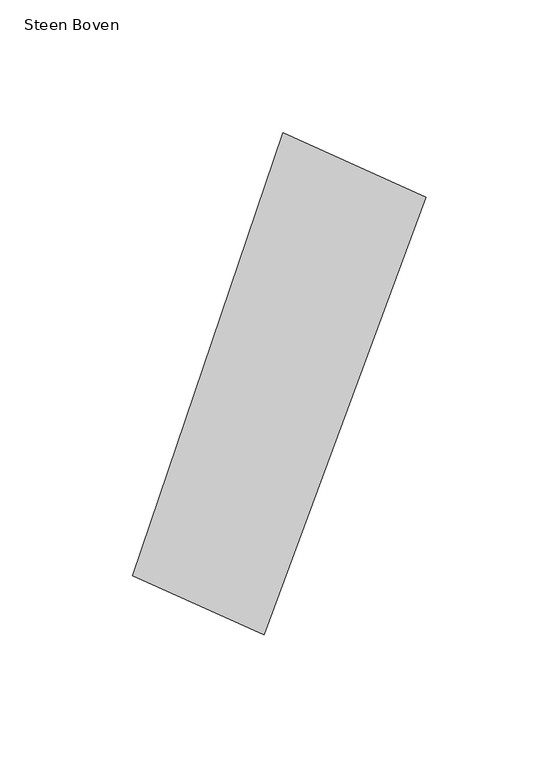
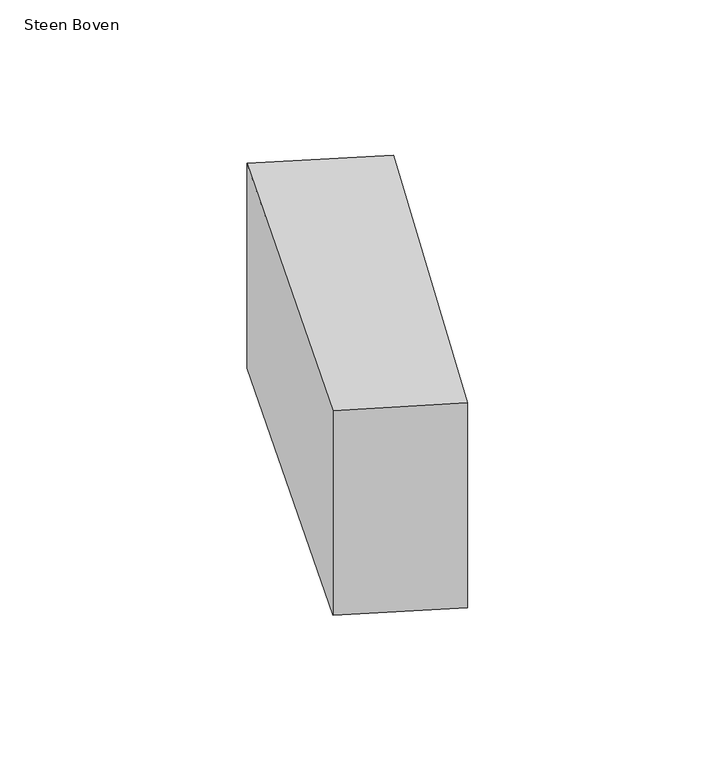
"""IFC4 building model written with IfcOpenShell, lengths in millimetres: proxy geometry, 00_GMA_steen_versie_4 : Steen Boven."""

from ifc_helpers import new_model, si_unit, origin, origin_with_axes, place, context, project, spatial, polyline, outline, extrude, source, transform, mapped, element, save


def steen_boven_4d50c7ad(model_context):
    return source(origin(), model_context, "Body", "SweptSolid", [
        extrude(outline(polyline([(132.3373334, 155.2461743), (71.3898275, -9.2546964), (22.0359236, 12.9928738), (78.5853065, 179.4877053), (132.3373334, 155.2461743)])), origin_with_axes(), (0.0, 0.0, 1.0), 100.0),
    ])


if __name__ == "__main__":
    model = new_model("IFC4")
    model_context = context("Model", 3, world=origin())
    ifc_project = project(units=[si_unit("LENGTHUNIT", "METRE", prefix="MILLI")], contexts=[model_context])
    site = spatial("IfcSite", under=ifc_project)
    building = spatial("IfcBuilding", under=site)
    placement = place(None, origin())
    steen_boven_shape = steen_boven_4d50c7ad(model_context)
    element("IfcBuildingElementProxy", 1, Name="00_GMA_steen_versie_4 : Steen Boven", ObjectType="00_GMA_steen_versie_4 : Steen Boven", at=placement, inside=building, context=model_context, shape_type="MappedRepresentation", body=[
        mapped(steen_boven_shape, transform((0.0, 0.0, 0.0), x_axis=(1.0, 0.0, 0.0), y_axis=(0.0, 1.0, 0.0), z_axis=(0.0, 0.0, 1.0))),
    ])
    save(model, "model.ifc")

# Revit data of these elements
# Type "00_GMA_steen_versie_4 : Steen Boven"
#   StootVoegHalfBoven [instance default] = 5 mm
#   StootVoegHalf [instance default] = 5 mm
#   StootVoegBreedteOnder = 10 mm
#   StootVoegBreedteBoven = 10 mm
#   Steendikte = 100 mm
#   LintVoegOnderHalf = 5 mm
#   LintVoegOnder = 10 mm
#   LintVoegBovenHalf = 0 mm
#   LintVoegBoven = 0 mm
#   materiaal = none
#   MateriaalVoeg = none
#   Default Elevation = 0
